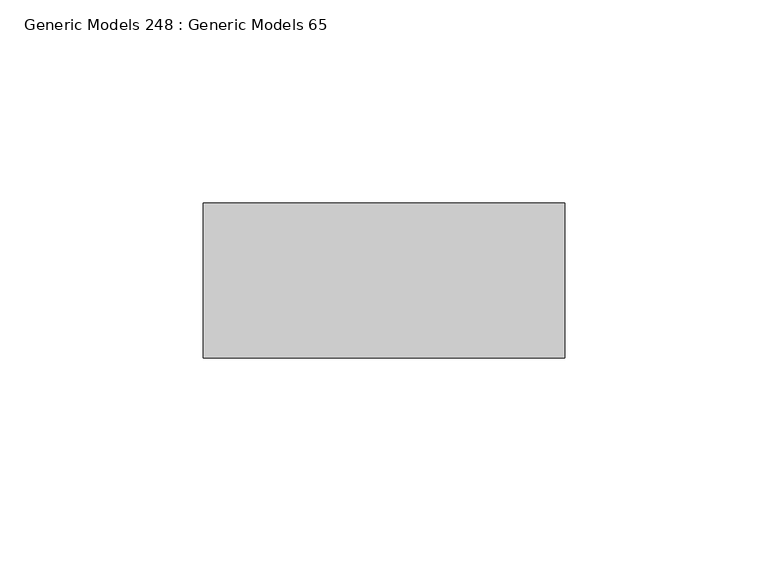
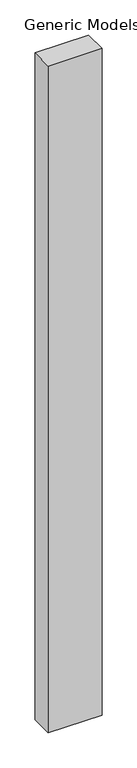
"""IFC4 building model written with IfcOpenShell, lengths in millimetres: proxy geometry, Generic Models 248 : Generic Models 65."""

from ifc_helpers import new_model, si_unit, frame, origin, place, context, project, spatial, polyline, outline, extrude, source, transform, mapped, element, save


def generic_models_248_generic_models_65_f6c484d7(model_context):
    return source(origin(), model_context, "Body", "SweptSolid", [
        extrude(outline(polyline([(47345.6, 592.1375), (47256.7, 592.1375), (47256.7, 630.2375), (47345.6, 630.2375), (47345.6, 592.1375)])), frame((0.0, 0.0, 4305.3), z_axis=(0.0, 0.0, 1.0), x_axis=(1.0, 0.0, 0.0)), (0.0, 0.0, 1.0), 1162.05),
    ])


if __name__ == "__main__":
    model = new_model("IFC4")
    model_context = context("Model", 3, world=origin())
    ifc_project = project(units=[si_unit("LENGTHUNIT", "METRE", prefix="MILLI")], contexts=[model_context])
    site = spatial("IfcSite", under=ifc_project)
    building = spatial("IfcBuilding", under=site)
    placement = place(None, origin())
    generic_models_248_generic_models_65_shape = generic_models_248_generic_models_65_f6c484d7(model_context)
    element("IfcBuildingElementProxy", 1, Name="Generic Models 248 : Generic Models 65", ObjectType="Generic Models 248 : Generic Models 65", at=placement, inside=building, context=model_context, shape_type="MappedRepresentation", body=[
        mapped(generic_models_248_generic_models_65_shape, transform((0.0, 0.0, 0.0), x_axis=(1.0, 0.0, 0.0), y_axis=(0.0, 1.0, 0.0), z_axis=(0.0, 0.0, 1.0))),
    ])
    save(model, "model.ifc")

# Revit data of these elements
# Element 1 (IfcBuildingElementProxy, "Generic Models 248 : Generic Models 65")
#   Materials on its faces: "2X WOOD STUD - SEE 'WALL TAG' & 'LAYER MATERIAL SCHEDULE' FOR SPACING & INSULATION TREATMENT, IF APPLICAPLE"
# Materials
#   "2X WOOD STUD - SEE 'WALL TAG' & 'LAYER MATERIAL SCHEDULE' FOR SPACING & INSULATION TREATMENT, IF APPLICAPLE": class "Wood", colour RGB 234 198 147, transparency 0, Description = "Pinus Echinata", Cost = 0
